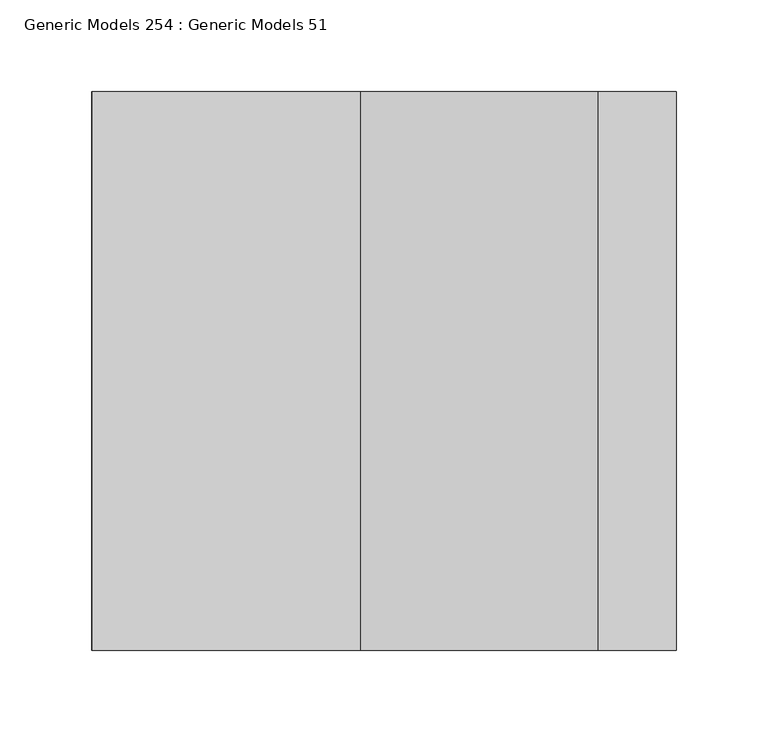
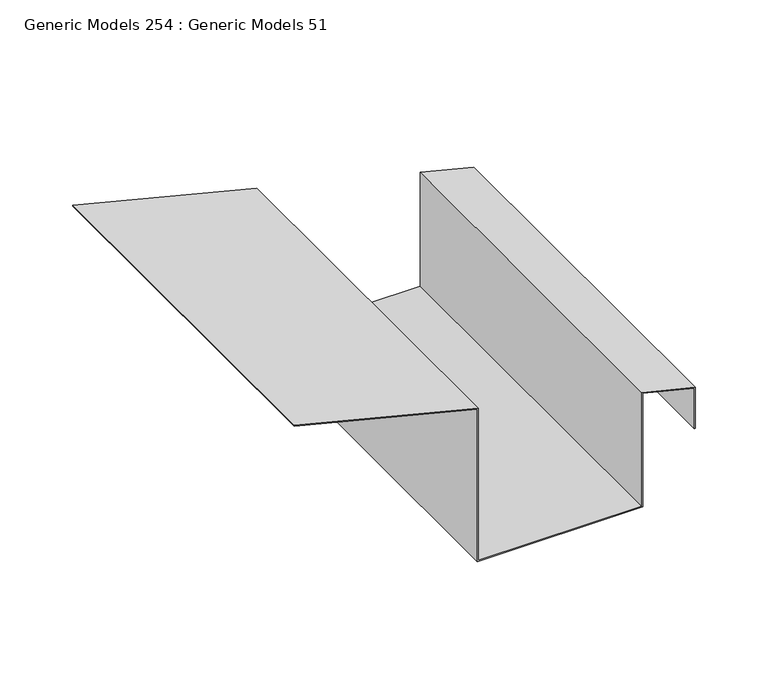
"""IFC4 building model written with IfcOpenShell, lengths in millimetres: proxy geometry, Generic Models 254 : Generic Models 51."""

from ifc_helpers import new_model, si_unit, frame, origin, place, context, project, spatial, polyline, outline, extrude, source, transform, mapped, element, save


def generic_models_254_generic_models_51_47aebbcd(model_context):
    return source(origin(), model_context, "Body", "SweptSolid", [
        extrude(outline(polyline([(127174.9344888, -31327.5556701), (127046.9095712, -31327.5556701), (127046.9095712, -31196.2089809), (127142.1595712, -31196.2089809), (127131.9086386, -31155.0947358), (127098.2529739, -31155.0947358), (127098.2529739, -31154.3009858), (127132.5287841, -31154.3009858), (127143.1755249, -31197.0027309), (127047.7033212, -31197.0027309), (127047.7033212, -31326.7619201), (127175.55423, -31326.7619201), (127212.0927928, -31472.9161713), (127211.3227422, -31473.108684), (127174.9344888, -31327.5556701)])), frame((0.0, 21665.9639348, 0.0), z_axis=(0.0, 1.0, 0.0), x_axis=(0.0, 0.0, 1.0)), (0.0, 0.0, 1.0), 304.8),
    ])


if __name__ == "__main__":
    model = new_model("IFC4")
    model_context = context("Model", 3, world=origin())
    ifc_project = project(units=[si_unit("LENGTHUNIT", "METRE", prefix="MILLI")], contexts=[model_context])
    site = spatial("IfcSite", under=ifc_project)
    building = spatial("IfcBuilding", under=site)
    placement = place(None, origin())
    generic_models_254_generic_models_51_shape = generic_models_254_generic_models_51_47aebbcd(model_context)
    element("IfcBuildingElementProxy", 1, Name="Generic Models 254 : Generic Models 51", ObjectType="Generic Models 254 : Generic Models 51", at=placement, inside=building, context=model_context, shape_type="MappedRepresentation", body=[
        mapped(generic_models_254_generic_models_51_shape, transform((0.0, 0.0, 0.0), x_axis=(1.0, 0.0, 0.0), y_axis=(0.0, 1.0, 0.0), z_axis=(0.0, 0.0, 1.0))),
    ])
    save(model, "model.ifc")

# Revit data of these elements
# Element 1 (IfcBuildingElementProxy, "Generic Models 254 : Generic Models 51")
#   Materials on its faces: "_SELF ADHERED MEMBRANE"
# Materials
#   "_SELF ADHERED MEMBRANE": class "Generic", colour RGB 253 192 103, transparency 0, Cost = 0
